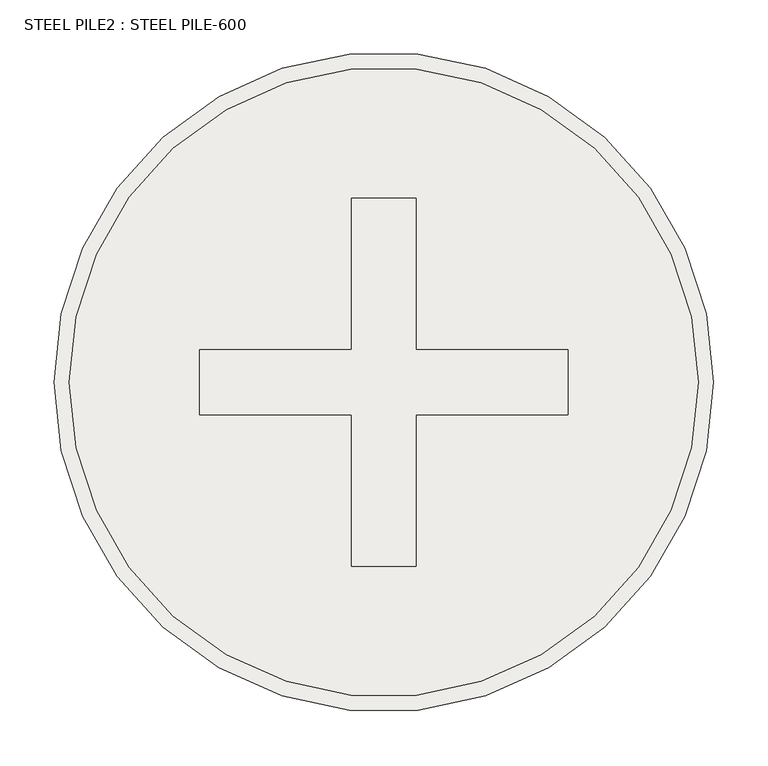
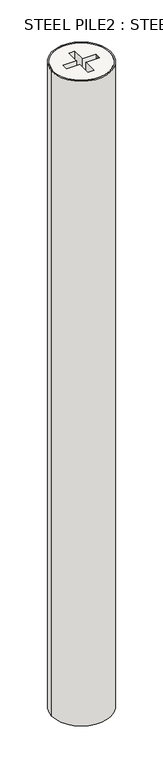
"""IFC4 building model written with IfcOpenShell, lengths in millimetres: slab geometry, STEEL PILE2 : STEEL PILE-600."""

from ifc_helpers import new_model, si_unit, point, frame, frame_2d, origin, place, context, project, spatial, circle_curve, trimmed, segment, composite_curve, outline, extrude, source, transform, mapped, element, save
from ifc_brep_helpers import plane_surface, cylinder_surface, advanced_brep


def steel_pile2_steel_pile_600_63b8d113(model_context):
    return source(origin(), model_context, "Body", "SolidModel", [
        advanced_brep(
        [(-290.5, 25499.5208589, 150.0), (290.5, 25499.5208589, 150.0), (-30.0, 25469.5208589, 150.0), (-170.0, 25469.5208589, 150.0), (-170.0, 25499.5208589, 150.0), (-170.0, 25529.5208589, 150.0), (-30.0, 25529.5208589, 150.0), (-30.0, 25669.5208589, 150.0), (30.0, 25669.5208589, 150.0), (30.0, 25529.5208589, 150.0), (170.0, 25529.5208589, 150.0), (170.0, 25499.5208589, 150.0), (170.0, 25469.5208589, 150.0), (30.0, 25469.5208589, 150.0), (30.0, 25329.5208589, 150.0), (-30.0, 25329.5208589, 150.0), (-290.5, 25499.5208589, -1850.0), (290.5, 25499.5208589, -1850.0), (-170.0, 25469.5208589, -160.0), (-30.0, 25469.5208589, -160.0), (-30.0, 25329.5208589, -160.0), (30.0, 25329.5208589, -160.0), (30.0, 25469.5208589, -160.0), (170.0, 25469.5208589, -160.0), (170.0, 25499.5208589, -160.0), (170.0, 25529.5208589, -160.0), (30.0, 25529.5208589, -160.0), (30.0, 25669.5208589, -160.0), (-30.0, 25669.5208589, -160.0), (-30.0, 25529.5208589, -160.0), (-170.0, 25529.5208589, -160.0), (-170.0, 25499.5208589, -160.0)],
        [
            (0, 1, circle_curve(frame((0.0, 25499.5208589, 150.0), z_axis=(0.0, 0.0, 1.0), x_axis=(1.0, 0.0, 0.0)), 290.5)),
            (1, 0, circle_curve(frame((0.0, 25499.5208589, 150.0), z_axis=(0.0, 0.0, 1.0), x_axis=(1.0, 0.0, 0.0)), 290.5)),
            (2, 3),
            (3, 4),
            (4, 5),
            (5, 6),
            (6, 7),
            (7, 8),
            (8, 9),
            (9, 10),
            (10, 11),
            (11, 12),
            (12, 13),
            (13, 14),
            (14, 15),
            (15, 2),
            (16, 17, circle_curve(frame((0.0, 25499.5208589, -1850.0), z_axis=(0.0, 0.0, -1.0), x_axis=(1.0, 0.0, 0.0)), 290.5)),
            (17, 16, circle_curve(frame((0.0, 25499.5208589, -1850.0), z_axis=(0.0, 0.0, -1.0), x_axis=(1.0, 0.0, 0.0)), 290.5)),
            (0, 16),
            (17, 1),
            (18, 19),
            (19, 20),
            (20, 21),
            (21, 22),
            (22, 23),
            (23, 24),
            (24, 25),
            (25, 26),
            (26, 27),
            (27, 28),
            (28, 29),
            (29, 30),
            (30, 31),
            (31, 18),
            (18, 3),
            (2, 19),
            (15, 20),
            (14, 21),
            (13, 22),
            (12, 23),
            (11, 24),
            (10, 25),
            (9, 26),
            (8, 27),
            (7, 28),
            (6, 29),
            (5, 30),
            (4, 31),
        ],
        [
            plane_surface(frame((290.5, 25499.5208589, 150.0), z_axis=(0.0, 0.0, 1.0), x_axis=(0.0, 1.0, 0.0))),
            plane_surface(frame((290.5, 25499.5208589, -1850.0), z_axis=(0.0, 0.0, -1.0), x_axis=(0.0, -1.0, 0.0))),
            cylinder_surface(frame((0.0, 25499.5208589, -1850.0), z_axis=(0.0, 0.0, 1.0), x_axis=(1.0, 0.0, 0.0)), 290.5),
            plane_surface(frame((-170.0, 25469.5208589, -160.0), z_axis=(0.0, 0.0, 1.0), x_axis=(-1.0, 0.0, 0.0))),
            plane_surface(frame((-170.0, 25469.5208589, 160.0), z_axis=(0.0, 1.0, 0.0), x_axis=(0.0, 0.0, -1.0))),
            plane_surface(frame((-30.0, 25469.5208589, 160.0), z_axis=(1.0, 0.0, 0.0), x_axis=(0.0, 0.0, -1.0))),
            plane_surface(frame((-30.0, 25329.5208589, 160.0), z_axis=(0.0, 1.0, 0.0), x_axis=(0.0, 0.0, -1.0))),
            plane_surface(frame((30.0, 25329.5208589, 160.0), z_axis=(-1.0, 0.0, 0.0), x_axis=(0.0, 0.0, -1.0))),
            plane_surface(frame((30.0, 25469.5208589, 160.0), z_axis=(0.0, 1.0, 0.0), x_axis=(0.0, 0.0, -1.0))),
            plane_surface(frame((170.0, 25469.5208589, 160.0), z_axis=(-1.0, 0.0, 0.0), x_axis=(0.0, 0.0, -1.0))),
            plane_surface(frame((170.0, 25499.5208589, 160.0), z_axis=(-1.0, 0.0, 0.0), x_axis=(0.0, 0.0, -1.0))),
            plane_surface(frame((170.0, 25529.5208589, 160.0), z_axis=(0.0, -1.0, 0.0), x_axis=(0.0, 0.0, -1.0))),
            plane_surface(frame((30.0, 25529.5208589, 160.0), z_axis=(-1.0, 0.0, 0.0), x_axis=(0.0, 0.0, -1.0))),
            plane_surface(frame((30.0, 25669.5208589, 160.0), z_axis=(0.0, -1.0, 0.0), x_axis=(0.0, 0.0, -1.0))),
            plane_surface(frame((-30.0, 25669.5208589, 160.0), z_axis=(1.0, 0.0, 0.0), x_axis=(0.0, 0.0, -1.0))),
            plane_surface(frame((-30.0, 25529.5208589, 160.0), z_axis=(0.0, -1.0, 0.0), x_axis=(0.0, 0.0, -1.0))),
            plane_surface(frame((-170.0, 25529.5208589, 160.0), z_axis=(1.0, 0.0, 0.0), x_axis=(0.0, 0.0, -1.0))),
            plane_surface(frame((-170.0, 25499.5208589, 160.0), z_axis=(1.0, 0.0, 0.0), x_axis=(0.0, 0.0, -1.0))),
        ],
        [
            (0, [[1, 2], [3, 4, 5, 6, 7, 8, 9, 10, 11, 12, 13, 14, 15, 16]]),
            (1, [[17, 18]]),
            (2, [[-1, 19, -18, 20]]),
            (2, [[-2, -20, -17, -19]]),
            (3, [[21, 22, 23, 24, 25, 26, 27, 28, 29, 30, 31, 32, 33, 34]]),
            (4, [[-21, 35, -3, 36]]),
            (5, [[-22, -36, -16, 37]]),
            (6, [[-23, -37, -15, 38]]),
            (7, [[-24, -38, -14, 39]]),
            (8, [[-25, -39, -13, 40]]),
            (9, [[-26, -40, -12, 41]]),
            (10, [[-27, -41, -11, 42]]),
            (11, [[-28, -42, -10, 43]]),
            (12, [[-29, -43, -9, 44]]),
            (13, [[-30, -44, -8, 45]]),
            (14, [[-31, -45, -7, 46]]),
            (15, [[-32, -46, -6, 47]]),
            (16, [[-33, -47, -5, 48]]),
            (17, [[-34, -48, -4, -35]]),
        ],
    ),
        extrude(outline(composite_curve([segment(trimmed(circle_curve(frame_2d((0.0, 25499.5208589)), 304.5), [point((-304.5, 25499.5208589))], [point((304.5, 25499.5208589))], False, "CARTESIAN"), True, "CONTINUOUS"), segment(trimmed(circle_curve(frame_2d((0.0, 25499.5208589)), 304.5), [point((304.5, 25499.5208589))], [point((-304.5, 25499.5208589))], False, "CARTESIAN"), True, "CONTINUOUS")], self_intersect=False), holes=[composite_curve([segment(trimmed(circle_curve(frame_2d((0.0, 25499.5208589)), 290.5), [point((-290.5, 25499.5208589))], [point((290.5, 25499.5208589))], True, "CARTESIAN"), True, "CONTINUOUS"), segment(trimmed(circle_curve(frame_2d((0.0, 25499.5208589)), 290.5), [point((290.5, 25499.5208589))], [point((-290.5, 25499.5208589))], True, "CARTESIAN"), True, "CONTINUOUS")], self_intersect=False)]), frame((0.0, 0.0, -6850.0), z_axis=(0.0, 0.0, 1.0), x_axis=(1.0, 0.0, 0.0)), (0.0, 0.0, 1.0), 7000.0),
    ])


if __name__ == "__main__":
    model = new_model("IFC4")
    model_context = context("Model", 3, world=origin())
    ifc_project = project(units=[si_unit("LENGTHUNIT", "METRE", prefix="MILLI")], contexts=[model_context])
    site = spatial("IfcSite", under=ifc_project)
    building = spatial("IfcBuilding", under=site)
    placement = place(None, origin())
    steel_pile2_steel_pile_600_shape = steel_pile2_steel_pile_600_63b8d113(model_context)
    element("IfcSlab", 1, ObjectType="STEEL PILE2 : STEEL PILE-600", at=placement, inside=building, context=model_context, shape_type="MappedRepresentation", body=[
        mapped(steel_pile2_steel_pile_600_shape, transform((0.0, 0.0, 0.0), x_axis=(1.0, 0.0, 0.0), y_axis=(0.0, 1.0, 0.0), z_axis=(0.0, 0.0, 1.0))),
    ])
    save(model, "model.ifc")
